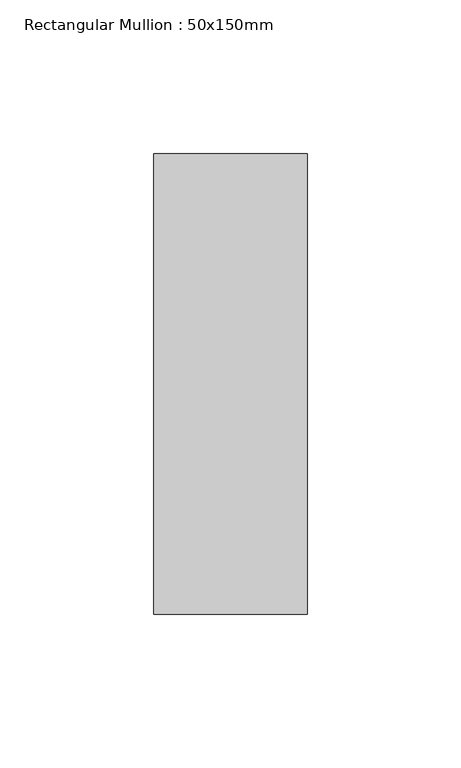
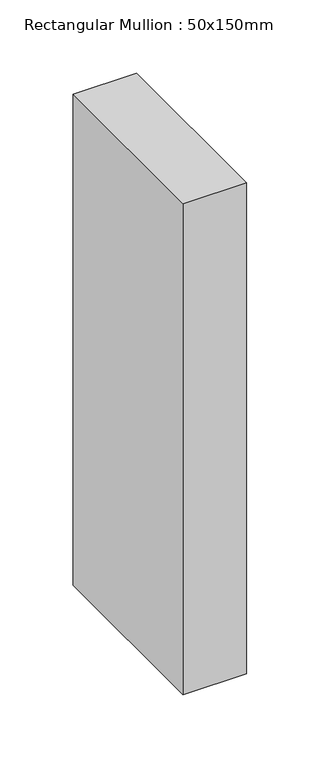
"""IFC4 building model written with IfcOpenShell, lengths in millimetres: member geometry, Rectangular Mullion : 50x150mm."""

from ifc_helpers import new_model, si_unit, frame, origin, place, context, project, spatial, polyline, outline, extrude, source, transform, mapped, element, save


def rectangular_mullion_50x150mm_11069a19(model_context):
    return source(origin(), model_context, "Body", "SweptSolid", [
        extrude(outline(polyline([(0.0, 75.0), (0.0, -75.0), (-50.0, -75.0), (-50.0, 75.0), (0.0, 75.0)])), frame((0.0, 0.0, -408.4078806), z_axis=(0.0, 0.0, 1.0), x_axis=(1.0, 0.0, 0.0)), (0.0, 0.0, 1.0), 408.4078806),
    ])


if __name__ == "__main__":
    model = new_model("IFC4")
    model_context = context("Model", 3, world=origin())
    ifc_project = project(units=[si_unit("LENGTHUNIT", "METRE", prefix="MILLI")], contexts=[model_context])
    site = spatial("IfcSite", under=ifc_project)
    building = spatial("IfcBuilding", under=site)
    placement = place(None, origin())
    rectangular_mullion_50x150mm_shape = rectangular_mullion_50x150mm_11069a19(model_context)
    element("IfcMember", 1, ObjectType="Rectangular Mullion : 50x150mm", at=placement, inside=building, context=model_context, shape_type="MappedRepresentation", body=[
        mapped(rectangular_mullion_50x150mm_shape, transform((0.0, 0.0, 0.0), x_axis=(1.0, 0.0, 0.0), y_axis=(0.0, 1.0, 0.0), z_axis=(0.0, 0.0, 1.0))),
    ])
    save(model, "model.ifc")

# Revit data of these elements
# Type "Rectangular Mullion : 50x150mm"
#   Keynote = "H11"
#   built-in parameter 1007304 = 0.492126 (stored number, unit not read)
#   built-in parameter 1007301 = 0.082021 (stored number, unit not read)
#   built-in parameter 1007300 = 0.082021 (stored number, unit not read)
# Element 1 (IfcMember, "Rectangular Mullion : 50x150mm")
#   Materials on its faces: "Aluminium"
# Materials
#   "Aluminium": class "Metal", colour RGB 247 247 247, transparency 0, Description = "Aluminium 6061", Cost = 0
